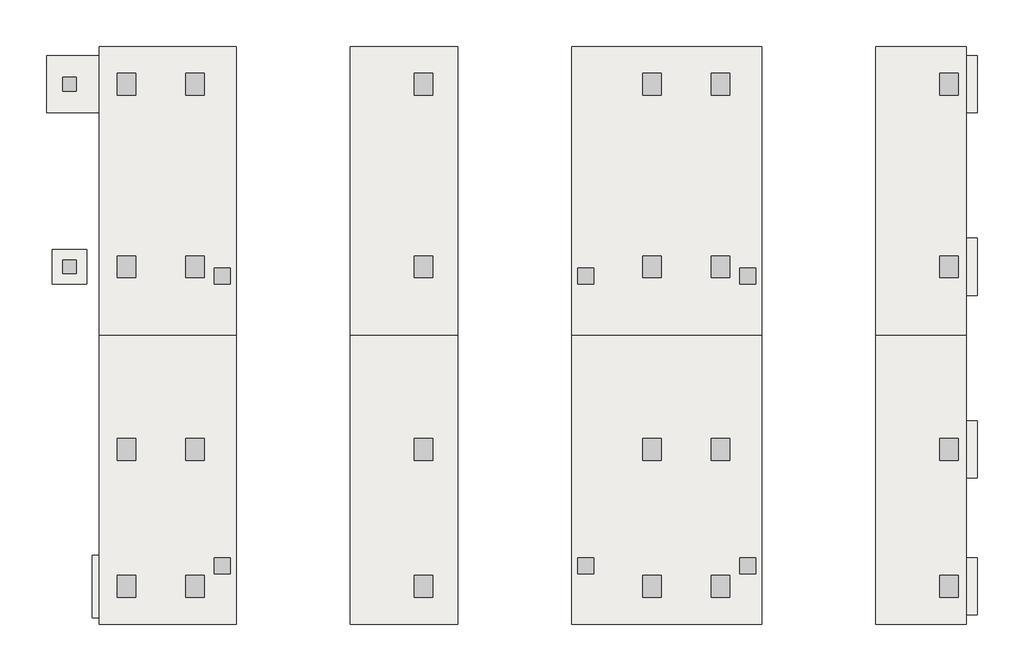
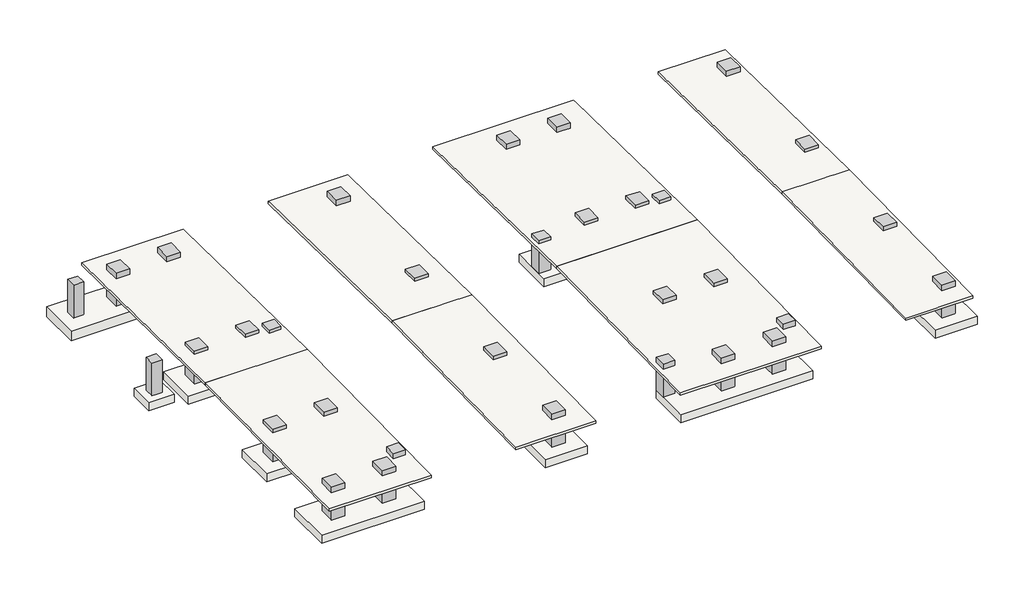
# Not in any storey: 32 columns, 25 slabs.
# Revit data of these elements (continued)
# Type "Footing-Rectangular_R1 : H_SF_AR_S18_W7800xL2740xT500_Bitumen_F9" (continued)
#   Width = 7800 mm
#   Length = 2500 mm
#   Foundation Thickness = 500 mm
#   Structural Material [instance default] = none
#   Assembly Code = ""
# Elements 1, 2, 3, 4, 5, 6, 7, 8, 9, 10, 11, 12, 13, 14, 15, 16, 17, 18, 19, 20, 21, 22, 23, 24 (IfcColumn, "RC_Column_Rectangular : H_SC_AR_S15_UG PED_W800xL950_Bit_PD1")
#   Comments = ""
#   hec_material3 = none
#   hec_material2 = none
#   hec_material1 = none
#   Structural Material = none
#   Phase Created = New Construction
# Elements 25, 26 (IfcColumn, "RC_Column_Rectangular : H_SC_AR_S15_UG PED_W600xL600_Bit_PD2")
#   Comments = ""
#   hec_material3 = none
#   hec_material2 = none
#   hec_material1 = none
#   Structural Material = none
#   Phase Created = New Construction
# Elements 27, 28, 29, 30, 31, 32 (IfcColumn, "RC_Column_Rectangular : H_SC_AR_S15_UG PED_W700xL700_Bit_PD3")
#   Comments = ""
#   hec_material3 = none
#   hec_material2 = none
#   hec_material1 = none
#   Structural Material = none
#   Phase Created = New Construction
# Elements 33, 35, 37, 40 (IfcSlab, "H_SF_AR_S17_SOG T150")
#   Comments = ""
#   Height Offset From Level = 0 mm
#   built-in parameter 1001954 = 1
#   Phase Created = New Construction
# Elements 34, 39 (IfcSlab, "H_SF_AR_S17_SOG T150")
#   Comments = ""
#   built-in parameter 1001955 = 3.14159 (stored number, unit not read)
#   Height Offset From Level = 0 mm
#   built-in parameter 1001954 = 1
#   Phase Created = New Construction
# Elements 36, 38 (IfcSlab, "H_SF_AR_S17_SOG T150")
#   Comments = ""
#   built-in parameter 1001955 = 1.5708 (stored number, unit not read)
#   Height Offset From Level = 0 mm
#   built-in parameter 1001954 = 1
#   Phase Created = New Construction
# Elements 41, 42, 43, 44, 45, 46, 47, 48 (IfcSlab, "Footing-Rectangular_R1 : H_SF_AR_S18_W2500xL2500xT500_Bitumen_F1")
#   Comments = ""
#   Structural Material = none
#   Phase Created = New Construction
# Element 49 (IfcSlab, "Footing-Rectangular_R1 : H_SF_AR_S18_W1500xL1500xT500_Bitumen_F2")
#   Comments = ""
#   Structural Material = none
#   Phase Created = New Construction
# Elements 50, 51 (IfcSlab, "Footing-Rectangular_R1 : H_SF_AR_S18_W5400xL2500xT500_Bitumen_F3")
#   Comments = ""
#   Structural Material = none
#   Phase Created = New Construction
# Element 52 (IfcSlab, "Footing-Rectangular_R1 : H_SF_AR_S18_W6000xL2500xT500_Bitumen_F4")
#   Comments = ""
#   Structural Material = none
#   Phase Created = New Construction
# Element 53 (IfcSlab, "Footing-Rectangular_R1 : H_SF_AR_S18_W8000xL2500xT500_Bitumen_F5")
#   Comments = ""
#   Structural Material = none
#   Phase Created = New Construction
# Element 54 (IfcSlab, "Footing-Rectangular_R1 : H_SF_AR_S18_W5750xL2500xT500_Bitumen_F6")
#   Comments = ""
#   Structural Material = none
#   Phase Created = New Construction
# Element 55 (IfcSlab, "Footing-Rectangular_R1 : H_SF_AR_S18_W7800xL2500xT500_Bitumen_F7")
#   Comments = ""
#   Structural Material = none
#   Phase Created = New Construction
# Element 56 (IfcSlab, "Footing-Rectangular_R1 : H_SF_AR_S18_W6050xL2740xT500_Bitumen_F8")
#   Comments = ""
#   Structural Material = none
#   Phase Created = New Construction
# Element 57 (IfcSlab, "Footing-Rectangular_R1 : H_SF_AR_S18_W7800xL2740xT500_Bitumen_F9")
#   Comments = ""
#   Structural Material = none
#   Phase Created = New Construction
